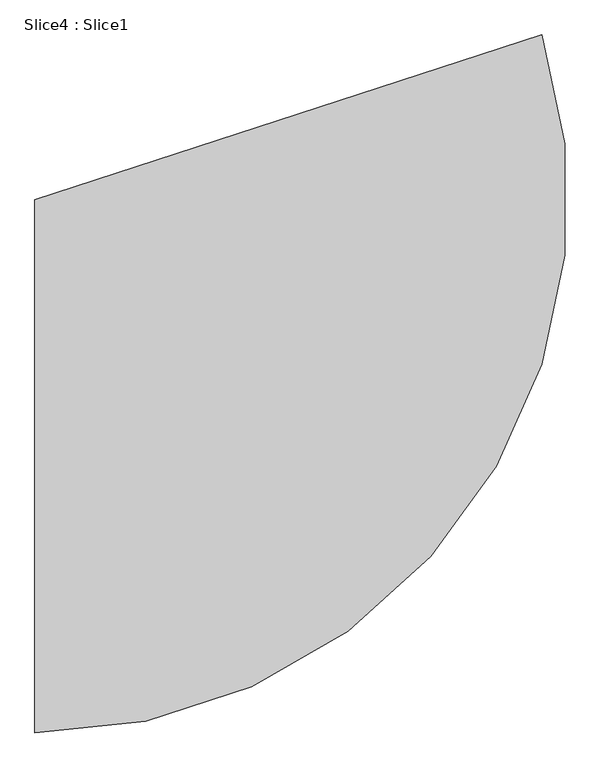
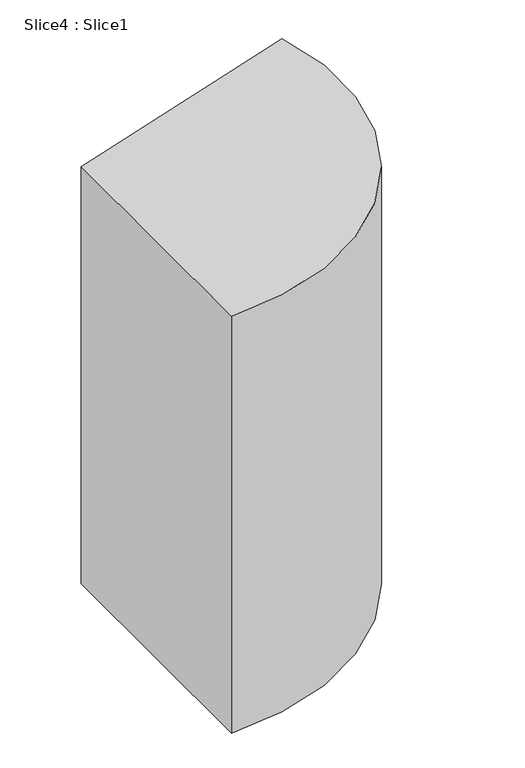
"""IFC4 building model written with IfcOpenShell, lengths in millimetres: proxy geometry, Slice4 : Slice1."""

from ifc_helpers import new_model, si_unit, point, origin, origin_with_axes, origin_2d, place, context, project, spatial, polyline, circle_curve, trimmed, segment, composite_curve, outline, extrude, source, transform, mapped, element, save


def slice4_slice1_723c6fc5(model_context):
    return source(origin(), model_context, "Body", "SweptSolid", [
        extrude(outline(composite_curve([segment(polyline([(0.0, -1100.0), (0.0, 0.0), (1046.1621679, 339.9186938)]), True, "CONTINUOUS"), segment(trimmed(circle_curve(origin_2d(), 1100.0), [point((1046.1621679, 339.9186938))], [point((0.0, -1100.0))], False, "CARTESIAN"), True, "CONTINUOUS")], self_intersect=False)), origin_with_axes(), (0.0, 0.0, 1.0), 1863.1990505),
    ])


if __name__ == "__main__":
    model = new_model("IFC4")
    model_context = context("Model", 3, world=origin())
    ifc_project = project(units=[si_unit("LENGTHUNIT", "METRE", prefix="MILLI")], contexts=[model_context])
    site = spatial("IfcSite", under=ifc_project)
    building = spatial("IfcBuilding", under=site)
    placement = place(None, origin())
    slice4_slice1_shape = slice4_slice1_723c6fc5(model_context)
    element("IfcBuildingElementProxy", 1, Name="Slice4 : Slice1", ObjectType="Slice4 : Slice1", at=placement, inside=building, context=model_context, shape_type="MappedRepresentation", body=[
        mapped(slice4_slice1_shape, transform((0.0, 0.0, 0.0), x_axis=(1.0, 0.0, 0.0), y_axis=(0.0, 1.0, 0.0), z_axis=(0.0, 0.0, 1.0))),
    ])
    save(model, "model.ifc")
